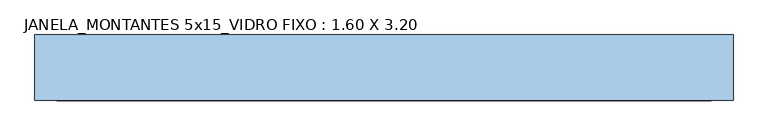
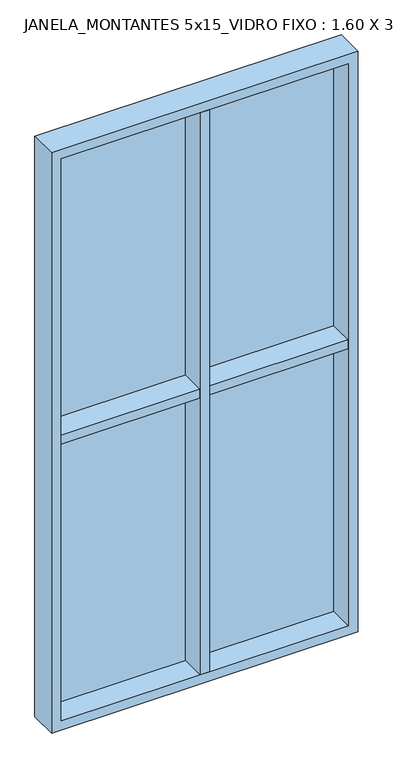
"""IFC4 building model written with IfcOpenShell, lengths in millimetres: window geometry, JANELA_MONTANTES 5x15_VIDRO FIXO : 1.60 X 3.20."""

from ifc_helpers import new_model, si_unit, frame, origin, place, context, project, spatial, polyline, outline, extrude, source, transform, mapped, element, save


def janela_montantes_5x15_vidro_fixo_1_60_x_3_20_cd7e8e18(model_context):
    return source(origin(), model_context, "Body", "SweptSolid", [
        extrude(outline(polyline([(750.0, 97.5), (750.0, -47.5), (-750.0, -47.5), (-750.0, 97.5), (750.0, 97.5)])), frame((0.0, 0.0, 2575.0), z_axis=(0.0, 0.0, 1.0), x_axis=(1.0, 0.0, 0.0)), (0.0, 0.0, 1.0), 50.0),
        extrude(outline(polyline([(25.0, 100.0), (25.0, -50.0), (-25.0, -50.0), (-25.0, 100.0), (25.0, 100.0)])), frame((0.0, 0.0, 1050.0), z_axis=(0.0, 0.0, 1.0), x_axis=(1.0, 0.0, 0.0)), (0.0, 0.0, 1.0), 3100.0),
        extrude(outline(polyline([(4200.0, -800.0), (1000.0, -800.0), (1000.0, 800.0), (4200.0, 800.0), (4200.0, -800.0)]), holes=[polyline([(4150.0, -750.0), (4150.0, 750.0), (1050.0, 750.0), (1050.0, -750.0), (4150.0, -750.0)])]), frame((0.0, -50.0, 0.0), z_axis=(0.0, 1.0, 0.0), x_axis=(0.0, 0.0, 1.0)), (0.0, 0.0, 1.0), 150.0),
        extrude(outline(polyline([(750.0, 80.0), (-750.0, 80.0), (-750.0, 92.0), (750.0, 92.0), (750.0, 80.0)])), frame((0.0, 0.0, 1050.0), z_axis=(0.0, 0.0, 1.0), x_axis=(1.0, 0.0, 0.0)), (0.0, 0.0, 1.0), 3100.0),
    ])


if __name__ == "__main__":
    model = new_model("IFC4")
    model_context = context("Model", 3, world=origin())
    ifc_project = project(units=[si_unit("LENGTHUNIT", "METRE", prefix="MILLI")], contexts=[model_context])
    site = spatial("IfcSite", under=ifc_project)
    building = spatial("IfcBuilding", under=site)
    placement = place(None, origin())
    janela_montantes_5x15_vidro_fixo_1_60_x_3_20_shape = janela_montantes_5x15_vidro_fixo_1_60_x_3_20_cd7e8e18(model_context)
    element("IfcWindow", 1, ObjectType="JANELA_MONTANTES 5x15_VIDRO FIXO : 1.60 X 3.20", at=placement, inside=building, context=model_context, shape_type="MappedRepresentation", body=[
        mapped(janela_montantes_5x15_vidro_fixo_1_60_x_3_20_shape, transform((0.0, 0.0, 0.0), x_axis=(1.0, 0.0, 0.0), y_axis=(0.0, 1.0, 0.0), z_axis=(0.0, 0.0, 1.0))),
    ])
    save(model, "model.ifc")

# Revit data of these elements
# Type "JANELA_MONTANTES 5x15_VIDRO FIXO : 1.60 X 3.20"
#   Type Mark = "J2"
#   Analytic Construction = "<Nenhum>"
#   Largura moldura = 0.10 m
#   Largura janela = 1.50 m
#   Espessura moldura = 0.03 m
#   Espaçamento montantes verticais [instance default] = 0.75 m
#   Espaçamento montantes horizontais [instance default] = 1.55 m
#   Altura janela = 3.10 m
#   Height = 3.20 m
#   Altura-padrão do peitoril = 1.00 m
#   Width = 1.60 m
#   N verticais [instance default] = 2
#   N horizontais [instance default] = 2
#   N de montantes verticais [instance default] = 1
#   N de montantes horizontais [instance default] = 1
#   Montate vertical vários [instance default] = no
#   Montante vertical único [instance default] = yes
#   Montante horizontal único [instance default] = yes
#   Montante horizontal vários [instance default] = no
#   Tipo de vidro = .VIDRO
#   Material da esquadria = .ALUMÍNIO COM PINTURA ELETROSTÁTICA BRANCA
#   Wall Closure = (empty or 0)
# Element 1 (IfcWindow, "JANELA_MONTANTES 5x15_VIDRO FIXO : 1.60 X 3.20")
#   Materials on its faces: ".ALUMÍNIO COM PINTURA ELETROSTÁTICA BRANCA", ".VIDRO"
# Materials
#   ".VIDRO": class "Genérico", colour RGB 198 236 255, transparency 0.95, Cost = 0
#   ".ALUMÍNIO COM PINTURA ELETROSTÁTICA BRANCA": class "CC_METAIS", colour RGB 241 241 241, transparency 0, Cost = 0
